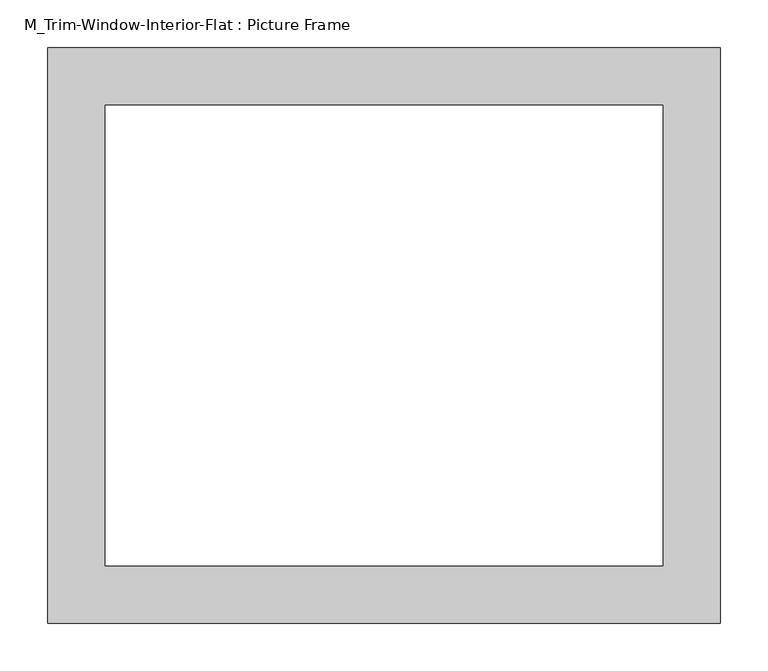
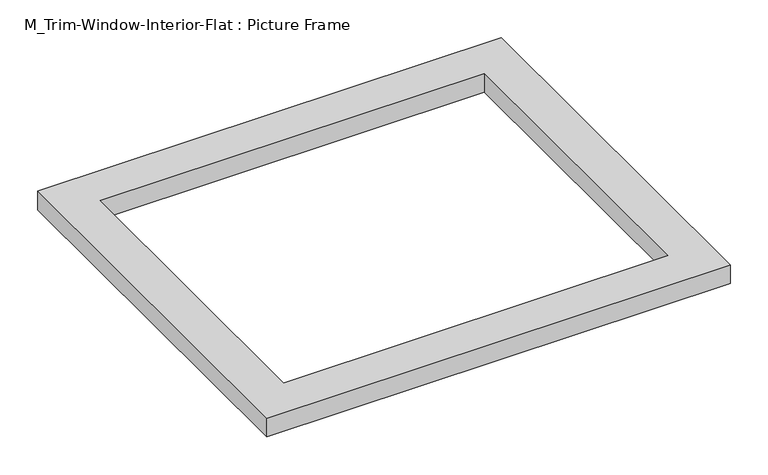
"""IFC4 building model written with IfcOpenShell, lengths in millimetres: proxy geometry, M_Trim-Window-Interior-Flat : Picture Frame."""

from ifc_helpers import new_model, si_unit, origin, origin_with_axes, place, context, project, spatial, polyline, outline, extrude, source, transform, mapped, element, save


def m_trim_window_interior_flat_picture_frame_0299c259(model_context):
    return source(origin(), model_context, "Body", "SweptSolid", [
        extrude(outline(polyline([(352.1, -47.3), (-352.1, -47.3), (-352.1, 555.3), (352.1, 555.3), (352.1, -47.3)]), holes=[polyline([(292.1, 12.7), (292.1, 495.3), (-292.1, 495.3), (-292.1, 12.7), (292.1, 12.7)])]), origin_with_axes(), (0.0, 0.0, 1.0), 30.0),
    ])


if __name__ == "__main__":
    model = new_model("IFC4")
    model_context = context("Model", 3, world=origin())
    ifc_project = project(units=[si_unit("LENGTHUNIT", "METRE", prefix="MILLI")], contexts=[model_context])
    site = spatial("IfcSite", under=ifc_project)
    building = spatial("IfcBuilding", under=site)
    placement = place(None, origin())
    m_trim_window_interior_flat_picture_frame_shape = m_trim_window_interior_flat_picture_frame_0299c259(model_context)
    element("IfcBuildingElementProxy", 1, Name="M_Trim-Window-Interior-Flat : Picture Frame", ObjectType="M_Trim-Window-Interior-Flat : Picture Frame", at=placement, inside=building, context=model_context, shape_type="MappedRepresentation", body=[
        mapped(m_trim_window_interior_flat_picture_frame_shape, transform((0.0, 0.0, 0.0), x_axis=(1.0, 0.0, 0.0), y_axis=(0.0, 1.0, 0.0), z_axis=(0.0, 0.0, 1.0))),
    ])
    save(model, "model.ifc")

# Revit data of these elements
# Type "M_Trim-Window-Interior-Flat : Picture Frame"
#   Trim Thickness_Picture Frame = 0' - 1.1811"
#   Trim Width = 0' - 2.3622"
#   Trim Thickness_with Sill = 0' - 0.7874"
#   Sill Thickness = 0' - 1.1811"
#   Opening Width [instance default] = 1' - 11.62205"
#   Opening Height [instance default] = 2' - 11.43307"
#   Default Elevation = 3' - 11.24409"
#   Sill = no
#   Picture Frame = yes
#   Trim Material [instance default] = none
# Element 1 (IfcBuildingElementProxy, "M_Trim-Window-Interior-Flat : Picture Frame")
#   Opening Width = 2' - 0"
#   Opening Height = 1' - 8"
#   Trim Material = Wood - Stained
#   Materials on its faces: "Wood - Stained"
# Materials
#   "Wood - Stained": class "Wood", colour RGB 224 178 126, transparency 0, Cost = 0
